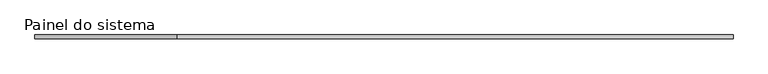
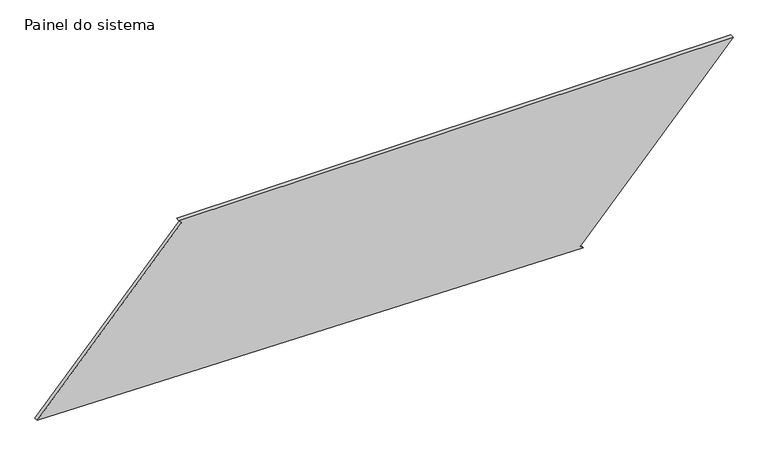
"""IFC4 building model written with IfcOpenShell, lengths in millimetres: plate geometry, Painel do sistema : Envidraçado."""

import ifcopenshell
import ifcopenshell.guid

model = None  # the IFC model being written
_history = None  # IfcOwnerHistory: only IFC2X3 demands one
_inside = {}  # id of a spatial element -> (the spatial element, [elements in it])
_under = {}  # id of a project, library or spatial element -> (it, [spatial elements below it])
_declared = {}  # id of a project -> (the project, [libraries it declares])
_typed = {}  # id of a type object -> (the type object, [elements of that type])
_made_of = {}  # id of a material, layer set ... -> (it, [elements and type objects made of it])


def new_model(schema):
    """Start an empty IFC model of exactly this schema.

    Asked for "IFC4X3", IfcOpenShell would pick the latest addendum, in which some entities
    have other attributes; the version numbers below select the first issue.
    IFC2X3 requires an IfcOwnerHistory on every rooted entity: one is made here for all.
    """
    global model, _history
    if schema == "IFC4X3":
        model = ifcopenshell.file(schema_version=(4, 3, 0, 0))
    else:
        model = ifcopenshell.file(schema=schema)
    _inside.clear()
    _under.clear()
    _declared.clear()
    _typed.clear()
    _made_of.clear()
    _history = None
    if model.schema == "IFC2X3":
        org = make("IfcOrganization", Name="unknown")
        user = make(
            "IfcPersonAndOrganization",
            ThePerson=make("IfcPerson", FamilyName="unknown"),
            TheOrganization=org,
        )
        app = make(
            "IfcApplication",
            ApplicationDeveloper=org,
            Version="unknown",
            ApplicationFullName="unknown",
            ApplicationIdentifier="unknown",
        )
        _history = make(
            "IfcOwnerHistory",
            OwningUser=user,
            OwningApplication=app,
            ChangeAction="ADDED",
            CreationDate=0,
        )
    return model


def make(cls, **values):
    """One entity of the class cls with the attributes given. An attribute that is None is left unset."""
    return model.create_entity(
        cls, **{name: value for name, value in values.items() if value is not None}
    )


def rooted(cls, **values):
    """An entity with a GlobalId (a new one), such as an element, a storey or a relation."""
    return make(cls, GlobalId=ifcopenshell.guid.new(), OwnerHistory=_history, **values)


def si_unit(unit_type, name, prefix=None):
    """IfcSIUnit, for example si_unit("LENGTHUNIT", "METRE", prefix="MILLI")."""
    return make("IfcSIUnit", UnitType=unit_type, Prefix=prefix, Name=name)


def assignment(units):
    """IfcUnitAssignment: the units of a project."""
    return None if units is None else make("IfcUnitAssignment", Units=units)


def point(xyz):
    """IfcCartesianPoint."""
    return None if xyz is None else make("IfcCartesianPoint", Coordinates=xyz)


def direction(xyz):
    """IfcDirection."""
    return None if xyz is None else make("IfcDirection", DirectionRatios=xyz)


def frame(location, z_axis=None, x_axis=None):
    """IfcAxis2Placement3D, a coordinate frame: its origin and axes. An axis left out is left unset."""
    return make(
        "IfcAxis2Placement3D",
        Location=point(location),
        Axis=direction(z_axis),
        RefDirection=direction(x_axis),
    )


def origin():
    """The frame at (0, 0, 0) with its axes left unset."""
    return frame((0.0, 0.0, 0.0))


def place(relative_to, where):
    """IfcLocalPlacement: puts the frame where relative to a parent placement (None: the world)."""
    return make(
        "IfcLocalPlacement", PlacementRelTo=relative_to, RelativePlacement=where
    )


def context(
    kind, dimensions, precision=None, world=None, true_north=None, identifier=None
):
    """IfcGeometricRepresentationContext, for example the 3D "Model" context."""
    return make(
        "IfcGeometricRepresentationContext",
        ContextIdentifier=identifier,
        ContextType=kind,
        CoordinateSpaceDimension=dimensions,
        Precision=precision,
        WorldCoordinateSystem=world,
        TrueNorth=true_north,
    )


def project(units=None, contexts=None):
    """IfcProject with its units and contexts."""
    return rooted(
        "IfcProject",
        Name="project",
        RepresentationContexts=contexts,
        UnitsInContext=assignment(units),
    )


def spatial(cls, under=None, at=None, **own):
    """A site, building, storey or space (cls), placed at a placement, below another one or the project."""
    s = rooted(cls, ObjectPlacement=at, **own)
    if under is not None:
        _under.setdefault(under.id(), (under, []))[1].append(s)
    return s


def polyline(points):
    """IfcPolyline through the points."""
    return make("IfcPolyline", Points=[point(p) for p in points])


def outline(outer, holes=None, kind="AREA"):
    """IfcArbitraryClosedProfileDef: a profile drawn as a closed curve; with holes, ...WithVoids."""
    if holes is None:
        return make("IfcArbitraryClosedProfileDef", ProfileType=kind, OuterCurve=outer)
    return make(
        "IfcArbitraryProfileDefWithVoids",
        ProfileType=kind,
        OuterCurve=outer,
        InnerCurves=holes,
    )


def extrude(swept, where, along, depth):
    """IfcExtrudedAreaSolid: the profile swept, set in the frame where, extruded along a direction by depth."""
    return make(
        "IfcExtrudedAreaSolid",
        SweptArea=swept,
        Position=where,
        ExtrudedDirection=direction(along),
        Depth=depth,
    )


def shape(context_of_items, identifier, shape_type, items):
    """IfcShapeRepresentation: the items that make up one representation, for example the "Body"."""
    return make(
        "IfcShapeRepresentation",
        ContextOfItems=context_of_items,
        RepresentationIdentifier=identifier,
        RepresentationType=shape_type,
        Items=items,
    )


def source(mapping_origin, context_of_items, identifier, shape_type, items):
    """IfcRepresentationMap: a shape defined once, which mapped items show again and again."""
    return make(
        "IfcRepresentationMap",
        MappingOrigin=mapping_origin,
        MappedRepresentation=shape(context_of_items, identifier, shape_type, items),
    )


def transform(
    local_origin,
    x_axis=None,
    y_axis=None,
    z_axis=None,
    scale=None,
    scale2=None,
    scale3=None,
    uniform=True,
):
    """IfcCartesianTransformationOperator3D, or its non-uniform kind. x_axis, y_axis, z_axis: its Axis1, 2, 3."""
    if uniform:
        return make(
            "IfcCartesianTransformationOperator3D",
            Axis1=direction(x_axis),
            Axis2=direction(y_axis),
            LocalOrigin=point(local_origin),
            Scale=scale,
            Axis3=direction(z_axis),
        )
    return make(
        "IfcCartesianTransformationOperator3DnonUniform",
        Axis1=direction(x_axis),
        Axis2=direction(y_axis),
        LocalOrigin=point(local_origin),
        Scale=scale,
        Axis3=direction(z_axis),
        Scale2=scale2,
        Scale3=scale3,
    )


def mapped(mapping_source, mapping_target):
    """IfcMappedItem: shows the shape of a source again, moved by a transform."""
    return make(
        "IfcMappedItem", MappingSource=mapping_source, MappingTarget=mapping_target
    )


def made_of(thing, what):
    """Note that an element or type object is made of a material, layer set ...; save() writes the relation."""
    if what is not None:
        _made_of.setdefault(what.id(), (what, []))[1].append(thing)
    return thing


def element(
    cls,
    number,
    at=None,
    inside=None,
    cuts=None,
    type_object=None,
    material=None,
    context=None,
    identifier="Body",
    shape_type=None,
    held_by="IfcProductDefinitionShape",
    body=None,
    shapes=None,
    **own,
):
    """One element of the class cls, such as IfcWall. Its Tag is "e" and its number.

    at: its placement. inside: the storey or other place that contains it. cuts: it is an
    opening in that element (IfcRelVoidsElement). A single representation is given by context,
    identifier, shape_type and body (its items); several are given by shapes. held_by: the class
    of the entity that holds the representations. save() writes the other relations.
    """
    e = rooted(cls, Tag="e%d" % number, ObjectPlacement=at, **own)
    if body is not None:
        shapes = [shape(context, identifier, shape_type, body)]
    if shapes is not None:
        e.Representation = make(held_by, Representations=shapes)
    if inside is not None:
        _inside.setdefault(inside.id(), (inside, []))[1].append(e)
    if cuts is not None:
        rooted(
            "IfcRelVoidsElement", RelatingBuildingElement=cuts, RelatedOpeningElement=e
        )
    if type_object is not None:
        _typed.setdefault(type_object.id(), (type_object, []))[1].append(e)
    return made_of(e, material)


def aggregate(whole, parts):
    """IfcRelAggregates: a whole, such as a stair, and the parts it consists of."""
    return rooted("IfcRelAggregates", RelatingObject=whole, RelatedObjects=parts)


def save(model, path):
    """Write the relations noted so far, then the file.

    IfcRelAggregates (storeys below a building ...), IfcRelContainedInSpatialStructure (elements
    in a storey), IfcRelDefinesByType, IfcRelAssociatesMaterial and IfcRelDeclares: one each for
    every whole, place, type object, material and project.
    """
    for whole, parts in _under.values():
        aggregate(whole, parts)
    for where, things in _inside.values():
        rooted(
            "IfcRelContainedInSpatialStructure",
            RelatedElements=things,
            RelatingStructure=where,
        )
    for kind, things in _typed.values():
        rooted("IfcRelDefinesByType", RelatedObjects=things, RelatingType=kind)
    for what, things in _made_of.values():
        rooted("IfcRelAssociatesMaterial", RelatedObjects=things, RelatingMaterial=what)
    for by, libraries in _declared.values():
        rooted("IfcRelDeclares", RelatingContext=by, RelatedDefinitions=libraries)
    model.write(path)


def painel_do_sistema_ad4f3c23(model_context):
    return source(origin(), model_context, "Body", "SweptSolid", [
        extrude(outline(polyline([(0.0, 1232.9752161), (16.8339598, 1214.4923106), (1058.6710523, 2163.3822845), (1058.6710523, -1282.5436464), (1041.8370925, -1264.0607409), (54.4238329, -2163.3822845), (0.0, 1232.9752161)])), frame((0.0, 24.5, 0.0), z_axis=(0.0, 1.0, 0.0), x_axis=(0.0, 0.0, 1.0)), (0.0, 0.0, 1.0), 25.0),
    ])


if __name__ == "__main__":
    model = new_model("IFC4")
    model_context = context("Model", 3, world=origin())
    ifc_project = project(units=[si_unit("LENGTHUNIT", "METRE", prefix="MILLI")], contexts=[model_context])
    site = spatial("IfcSite", under=ifc_project)
    building = spatial("IfcBuilding", under=site)
    placement = place(None, origin())
    painel_do_sistema_shape = painel_do_sistema_ad4f3c23(model_context)
    element("IfcPlate", 1, ObjectType="Painel do sistema : Envidraçado", at=placement, inside=building, context=model_context, shape_type="MappedRepresentation", body=[
        mapped(painel_do_sistema_shape, transform((0.0, 0.0, 0.0), x_axis=(1.0, 0.0, 0.0), y_axis=(0.0, 1.0, 0.0), z_axis=(0.0, 0.0, 1.0))),
    ])
    save(model, "model.ifc")

# Revit data of these elements
# Type "Painel do sistema : Envidraçado"
#   Construction Type Id = "GSP4R"
#   Analytic Construction = "Vidraça única Pilkington 1/8 pol"
#   Visual Light Transmittance = 0.9
#   Solar Heat Gain Coefficient = 0.86
#   Heat Transfer Coefficient (U) = 6.7069 W/(m²·K)
# Element 1 (IfcPlate, "Painel do sistema : Envidraçado")
#   Materials on its faces: "Vidro"
# Materials
#   "Vidro": class "Vidro", colour RGB 0 128 192, transparency 0.9, Description = "Vidro de sílica", Cost = 0
